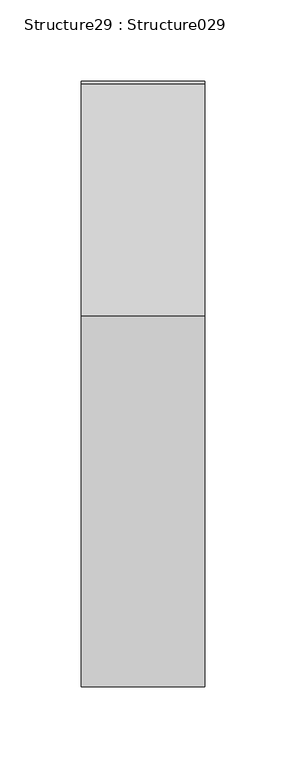
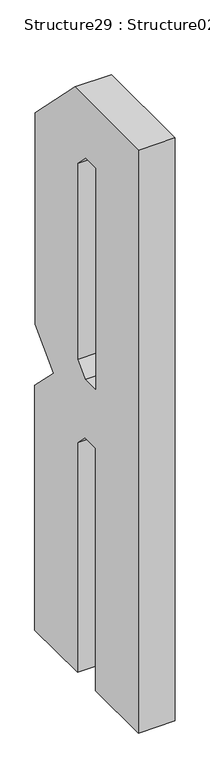
"""IFC4 building model written with IfcOpenShell, lengths in millimetres: proxy geometry, Structure29 : Structure029."""

import ifcopenshell
import ifcopenshell.guid

model = None  # the IFC model being written
_history = None  # IfcOwnerHistory: only IFC2X3 demands one
_inside = {}  # id of a spatial element -> (the spatial element, [elements in it])
_under = {}  # id of a project, library or spatial element -> (it, [spatial elements below it])
_declared = {}  # id of a project -> (the project, [libraries it declares])
_typed = {}  # id of a type object -> (the type object, [elements of that type])
_made_of = {}  # id of a material, layer set ... -> (it, [elements and type objects made of it])


def new_model(schema):
    """Start an empty IFC model of exactly this schema.

    Asked for "IFC4X3", IfcOpenShell would pick the latest addendum, in which some entities
    have other attributes; the version numbers below select the first issue.
    IFC2X3 requires an IfcOwnerHistory on every rooted entity: one is made here for all.
    """
    global model, _history
    if schema == "IFC4X3":
        model = ifcopenshell.file(schema_version=(4, 3, 0, 0))
    else:
        model = ifcopenshell.file(schema=schema)
    _inside.clear()
    _under.clear()
    _declared.clear()
    _typed.clear()
    _made_of.clear()
    _history = None
    if model.schema == "IFC2X3":
        org = make("IfcOrganization", Name="unknown")
        user = make(
            "IfcPersonAndOrganization",
            ThePerson=make("IfcPerson", FamilyName="unknown"),
            TheOrganization=org,
        )
        app = make(
            "IfcApplication",
            ApplicationDeveloper=org,
            Version="unknown",
            ApplicationFullName="unknown",
            ApplicationIdentifier="unknown",
        )
        _history = make(
            "IfcOwnerHistory",
            OwningUser=user,
            OwningApplication=app,
            ChangeAction="ADDED",
            CreationDate=0,
        )
    return model


def make(cls, **values):
    """One entity of the class cls with the attributes given. An attribute that is None is left unset."""
    return model.create_entity(
        cls, **{name: value for name, value in values.items() if value is not None}
    )


def rooted(cls, **values):
    """An entity with a GlobalId (a new one), such as an element, a storey or a relation."""
    return make(cls, GlobalId=ifcopenshell.guid.new(), OwnerHistory=_history, **values)


def si_unit(unit_type, name, prefix=None):
    """IfcSIUnit, for example si_unit("LENGTHUNIT", "METRE", prefix="MILLI")."""
    return make("IfcSIUnit", UnitType=unit_type, Prefix=prefix, Name=name)


def assignment(units):
    """IfcUnitAssignment: the units of a project."""
    return None if units is None else make("IfcUnitAssignment", Units=units)


def point(xyz):
    """IfcCartesianPoint."""
    return None if xyz is None else make("IfcCartesianPoint", Coordinates=xyz)


def direction(xyz):
    """IfcDirection."""
    return None if xyz is None else make("IfcDirection", DirectionRatios=xyz)


def frame(location, z_axis=None, x_axis=None):
    """IfcAxis2Placement3D, a coordinate frame: its origin and axes. An axis left out is left unset."""
    return make(
        "IfcAxis2Placement3D",
        Location=point(location),
        Axis=direction(z_axis),
        RefDirection=direction(x_axis),
    )


def origin():
    """The frame at (0, 0, 0) with its axes left unset."""
    return frame((0.0, 0.0, 0.0))


def place(relative_to, where):
    """IfcLocalPlacement: puts the frame where relative to a parent placement (None: the world)."""
    return make(
        "IfcLocalPlacement", PlacementRelTo=relative_to, RelativePlacement=where
    )


def context(
    kind, dimensions, precision=None, world=None, true_north=None, identifier=None
):
    """IfcGeometricRepresentationContext, for example the 3D "Model" context."""
    return make(
        "IfcGeometricRepresentationContext",
        ContextIdentifier=identifier,
        ContextType=kind,
        CoordinateSpaceDimension=dimensions,
        Precision=precision,
        WorldCoordinateSystem=world,
        TrueNorth=true_north,
    )


def project(units=None, contexts=None):
    """IfcProject with its units and contexts."""
    return rooted(
        "IfcProject",
        Name="project",
        RepresentationContexts=contexts,
        UnitsInContext=assignment(units),
    )


def spatial(cls, under=None, at=None, **own):
    """A site, building, storey or space (cls), placed at a placement, below another one or the project."""
    s = rooted(cls, ObjectPlacement=at, **own)
    if under is not None:
        _under.setdefault(under.id(), (under, []))[1].append(s)
    return s


def polyline(points):
    """IfcPolyline through the points."""
    return make("IfcPolyline", Points=[point(p) for p in points])


def outline(outer, holes=None, kind="AREA"):
    """IfcArbitraryClosedProfileDef: a profile drawn as a closed curve; with holes, ...WithVoids."""
    if holes is None:
        return make("IfcArbitraryClosedProfileDef", ProfileType=kind, OuterCurve=outer)
    return make(
        "IfcArbitraryProfileDefWithVoids",
        ProfileType=kind,
        OuterCurve=outer,
        InnerCurves=holes,
    )


def extrude(swept, where, along, depth):
    """IfcExtrudedAreaSolid: the profile swept, set in the frame where, extruded along a direction by depth."""
    return make(
        "IfcExtrudedAreaSolid",
        SweptArea=swept,
        Position=where,
        ExtrudedDirection=direction(along),
        Depth=depth,
    )


def shape(context_of_items, identifier, shape_type, items):
    """IfcShapeRepresentation: the items that make up one representation, for example the "Body"."""
    return make(
        "IfcShapeRepresentation",
        ContextOfItems=context_of_items,
        RepresentationIdentifier=identifier,
        RepresentationType=shape_type,
        Items=items,
    )


def source(mapping_origin, context_of_items, identifier, shape_type, items):
    """IfcRepresentationMap: a shape defined once, which mapped items show again and again."""
    return make(
        "IfcRepresentationMap",
        MappingOrigin=mapping_origin,
        MappedRepresentation=shape(context_of_items, identifier, shape_type, items),
    )


def transform(
    local_origin,
    x_axis=None,
    y_axis=None,
    z_axis=None,
    scale=None,
    scale2=None,
    scale3=None,
    uniform=True,
):
    """IfcCartesianTransformationOperator3D, or its non-uniform kind. x_axis, y_axis, z_axis: its Axis1, 2, 3."""
    if uniform:
        return make(
            "IfcCartesianTransformationOperator3D",
            Axis1=direction(x_axis),
            Axis2=direction(y_axis),
            LocalOrigin=point(local_origin),
            Scale=scale,
            Axis3=direction(z_axis),
        )
    return make(
        "IfcCartesianTransformationOperator3DnonUniform",
        Axis1=direction(x_axis),
        Axis2=direction(y_axis),
        LocalOrigin=point(local_origin),
        Scale=scale,
        Axis3=direction(z_axis),
        Scale2=scale2,
        Scale3=scale3,
    )


def mapped(mapping_source, mapping_target):
    """IfcMappedItem: shows the shape of a source again, moved by a transform."""
    return make(
        "IfcMappedItem", MappingSource=mapping_source, MappingTarget=mapping_target
    )


def made_of(thing, what):
    """Note that an element or type object is made of a material, layer set ...; save() writes the relation."""
    if what is not None:
        _made_of.setdefault(what.id(), (what, []))[1].append(thing)
    return thing


def element(
    cls,
    number,
    at=None,
    inside=None,
    cuts=None,
    type_object=None,
    material=None,
    context=None,
    identifier="Body",
    shape_type=None,
    held_by="IfcProductDefinitionShape",
    body=None,
    shapes=None,
    **own,
):
    """One element of the class cls, such as IfcWall. Its Tag is "e" and its number.

    at: its placement. inside: the storey or other place that contains it. cuts: it is an
    opening in that element (IfcRelVoidsElement). A single representation is given by context,
    identifier, shape_type and body (its items); several are given by shapes. held_by: the class
    of the entity that holds the representations. save() writes the other relations.
    """
    e = rooted(cls, Tag="e%d" % number, ObjectPlacement=at, **own)
    if body is not None:
        shapes = [shape(context, identifier, shape_type, body)]
    if shapes is not None:
        e.Representation = make(held_by, Representations=shapes)
    if inside is not None:
        _inside.setdefault(inside.id(), (inside, []))[1].append(e)
    if cuts is not None:
        rooted(
            "IfcRelVoidsElement", RelatingBuildingElement=cuts, RelatedOpeningElement=e
        )
    if type_object is not None:
        _typed.setdefault(type_object.id(), (type_object, []))[1].append(e)
    return made_of(e, material)


def aggregate(whole, parts):
    """IfcRelAggregates: a whole, such as a stair, and the parts it consists of."""
    return rooted("IfcRelAggregates", RelatingObject=whole, RelatedObjects=parts)


def save(model, path):
    """Write the relations noted so far, then the file.

    IfcRelAggregates (storeys below a building ...), IfcRelContainedInSpatialStructure (elements
    in a storey), IfcRelDefinesByType, IfcRelAssociatesMaterial and IfcRelDeclares: one each for
    every whole, place, type object, material and project.
    """
    for whole, parts in _under.values():
        aggregate(whole, parts)
    for where, things in _inside.values():
        rooted(
            "IfcRelContainedInSpatialStructure",
            RelatedElements=things,
            RelatingStructure=where,
        )
    for kind, things in _typed.values():
        rooted("IfcRelDefinesByType", RelatedObjects=things, RelatingType=kind)
    for what, things in _made_of.values():
        rooted("IfcRelAssociatesMaterial", RelatedObjects=things, RelatingMaterial=what)
    for by, libraries in _declared.values():
        rooted("IfcRelDeclares", RelatingContext=by, RelatedDefinitions=libraries)
    model.write(path)


def structure29_structure029_ef6f32be(model_context):
    return source(origin(), model_context, "Body", "SweptSolid", [
        extrude(outline(polyline([(537.7723378, 0.0), (537.7723378, -153.6683614), (32.9112648, -153.6683614), (5.4719383, -181.1076879), (5.4719383, -219.5256255), (537.7723378, -219.5256255), (537.7723378, -373.1592526), (-742.6586858, -373.1592526), (-742.6586858, -144.514577), (-599.9909621, -1.8468533), (-135.3828194, -1.8468533), (-67.6914097, -67.6914096), (0.0, 0.0), (537.7723378, 0.0)]), holes=[polyline([(-124.3898063, -219.5256255), (-124.3898063, -182.9350561), (-151.8325215, -155.4923409), (-581.7062671, -155.4923409), (-609.1455937, -182.9316674), (-609.1455937, -219.5256255), (-124.3898063, -219.5256255)])]), frame((-35624.0862846, 277955.3744385, 5017.4387266), z_axis=(1.0, 0.0, 1.354250045437766e-12), x_axis=(1.354250045437766e-12, 0.0, -1.0)), (0.0, 0.0, 1.0), 76.2),
    ])


if __name__ == "__main__":
    model = new_model("IFC4")
    model_context = context("Model", 3, world=origin())
    ifc_project = project(units=[si_unit("LENGTHUNIT", "METRE", prefix="MILLI")], contexts=[model_context])
    site = spatial("IfcSite", under=ifc_project)
    building = spatial("IfcBuilding", under=site)
    placement = place(None, origin())
    structure29_structure029_shape = structure29_structure029_ef6f32be(model_context)
    element("IfcBuildingElementProxy", 1, Name="Structure29 : Structure029", ObjectType="Structure29 : Structure029", at=placement, inside=building, context=model_context, shape_type="MappedRepresentation", body=[
        mapped(structure29_structure029_shape, transform((0.0, 0.0, 0.0), x_axis=(1.0, 0.0, 0.0), y_axis=(0.0, 1.0, 0.0), z_axis=(0.0, 0.0, 1.0))),
    ])
    save(model, "model.ifc")

# Revit data of these elements
# Type "Structure29 : Structure029"
#   NameOverride = "Structure029"
# Element 1 (IfcBuildingElementProxy, "Structure29 : Structure029")
#   Materials on its faces: "BRUSHED ALUMINUM LETTERING"
# Materials
#   "BRUSHED ALUMINUM LETTERING": class "Unassigned", colour RGB 169 181 186, transparency 0, Cost = 0
